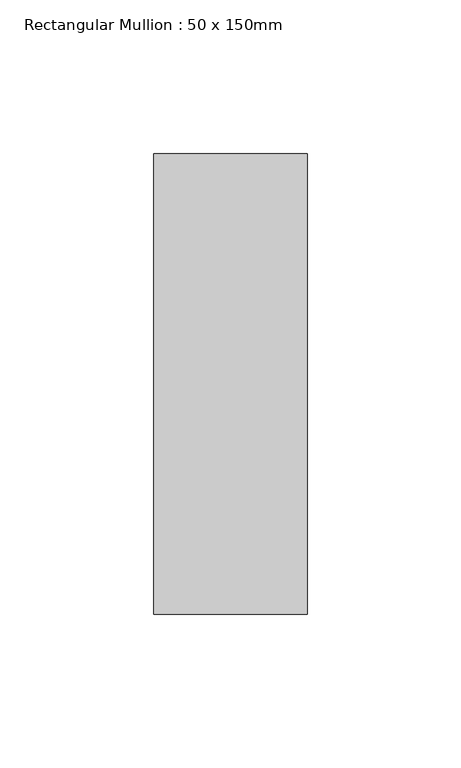
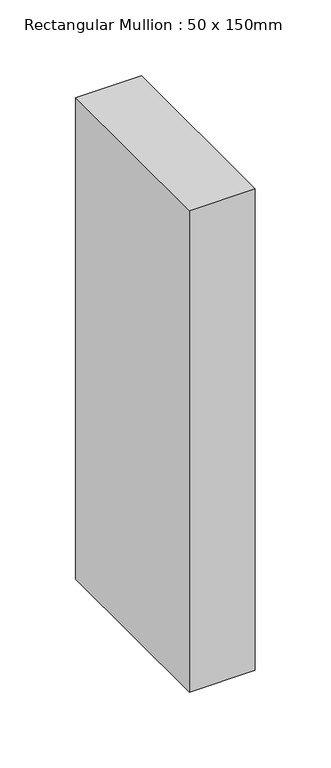
"""IFC4 building model written with IfcOpenShell, lengths in millimetres: member geometry, Rectangular Mullion : 50 x 150mm."""

from ifc_helpers import new_model, si_unit, frame, origin, place, context, project, spatial, polyline, outline, extrude, source, transform, mapped, element, save


def rectangular_mullion_50_x_150mm_ea2ffd58(model_context):
    return source(origin(), model_context, "Body", "SweptSolid", [
        extrude(outline(polyline([(25.0, 75.0), (25.0, -75.0), (-25.0, -75.0), (-25.0, 75.0), (25.0, 75.0)])), frame((0.0, 0.0, -387.5), z_axis=(0.0, 0.0, 1.0), x_axis=(1.0, 0.0, 0.0)), (0.0, 0.0, 1.0), 387.5),
    ])


if __name__ == "__main__":
    model = new_model("IFC4")
    model_context = context("Model", 3, world=origin())
    ifc_project = project(units=[si_unit("LENGTHUNIT", "METRE", prefix="MILLI")], contexts=[model_context])
    site = spatial("IfcSite", under=ifc_project)
    building = spatial("IfcBuilding", under=site)
    placement = place(None, origin())
    rectangular_mullion_50_x_150mm_shape = rectangular_mullion_50_x_150mm_ea2ffd58(model_context)
    element("IfcMember", 1, ObjectType="Rectangular Mullion : 50 x 150mm", at=placement, inside=building, context=model_context, shape_type="MappedRepresentation", body=[
        mapped(rectangular_mullion_50_x_150mm_shape, transform((0.0, 0.0, 0.0), x_axis=(1.0, 0.0, 0.0), y_axis=(0.0, 1.0, 0.0), z_axis=(0.0, 0.0, 1.0))),
    ])
    save(model, "model.ifc")

# Revit data of these elements
# Type "Rectangular Mullion : 50 x 150mm"
#   built-in parameter 1007304 = 0.492126 (stored number, unit not read)
#   built-in parameter 1007301 = 0.082021 (stored number, unit not read)
#   built-in parameter 1007300 = 0.082021 (stored number, unit not read)
# Element 1 (IfcMember, "Rectangular Mullion : 50 x 150mm")
#   Materials on its faces: "Aluminium"
# Materials
#   "Aluminium": class "Metal", colour RGB 247 247 247, transparency 0, Description = "Aluminium 6061", Cost = 0
